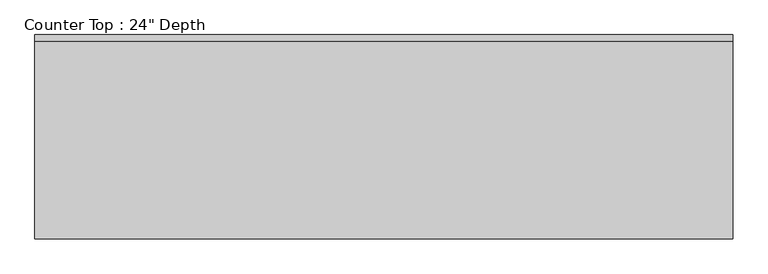
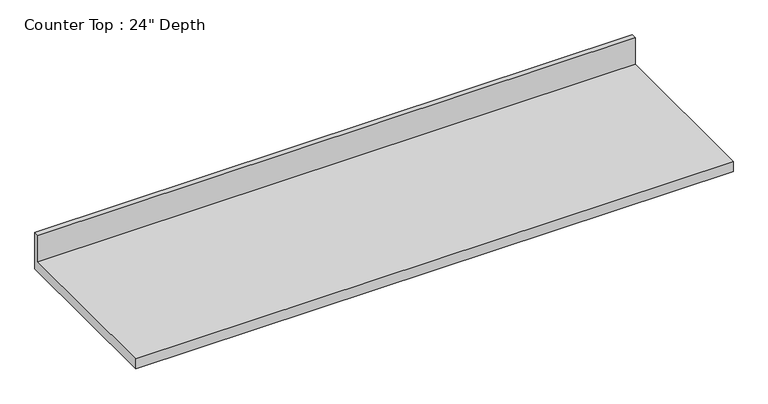
"""IFC4 building model written with IfcOpenShell, lengths in millimetres: furniture geometry."""

from ifc_helpers import new_model, si_unit, frame, origin, place, context, project, spatial, polyline, outline, extrude, source, transform, mapped, element, save


def furniture_b725675f(model_context):
    return source(origin(), model_context, "Body", "SweptSolid", [
        extrude(outline(polyline([(0.0, 1016.0), (0.0, 876.3), (-635.0, 876.3), (-635.0, 914.4), (-19.05, 914.4), (-19.05, 1016.0), (0.0, 1016.0)])), frame((-1200.4622951, 0.0, 0.0), z_axis=(1.0, 0.0, 0.0), x_axis=(0.0, 1.0, 0.0)), (0.0, 0.0, 1.0), 2168.525),
    ])


if __name__ == "__main__":
    model = new_model("IFC4")
    model_context = context("Model", 3, world=origin())
    ifc_project = project(units=[si_unit("LENGTHUNIT", "METRE", prefix="MILLI")], contexts=[model_context])
    site = spatial("IfcSite", under=ifc_project)
    building = spatial("IfcBuilding", under=site)
    placement = place(None, origin())
    furniture_shape = furniture_b725675f(model_context)
    element("IfcFurniture", 1, ObjectType="Counter Top : 24\" Depth", at=placement, inside=building, context=model_context, shape_type="MappedRepresentation", body=[
        mapped(furniture_shape, transform((0.0, 0.0, 0.0), x_axis=(1.0, 0.0, 0.0), y_axis=(0.0, 1.0, 0.0), z_axis=(0.0, 0.0, 1.0))),
    ])
    save(model, "model.ifc")

# Revit data of these elements
# Type "Counter Top : 24\" Depth"
#   Assembly Code = "C1030400"
#   Counter Thickness = 0' - 1 1/2"
#   Depth = 2' - 1"
#   Height = 3' - 0"
#   Length [instance default] = 8' - 0"
#   Counter Top Material = none
#   Default Elevation = 0
# Element 1 (IfcFurniture, "Counter Top : 24\" Depth")
#   Length = 7' - 1 3/8"
#   Materials on its faces: "Counter Top"
# Materials
#   "Counter Top": class "Wood", colour RGB 226 177 128, transparency 0
